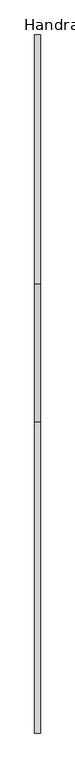
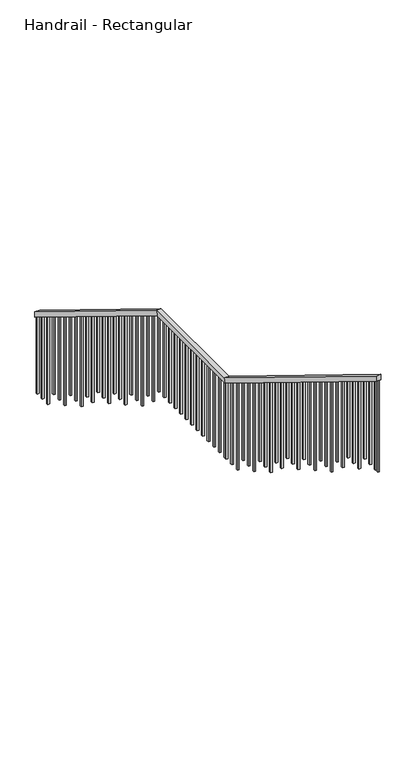
"""IFC4 building model written with IfcOpenShell, lengths in millimetres: railing geometry, Handrail - Rectangular."""

from ifc_helpers import new_model, si_unit, frame, origin, place, context, project, spatial, polyline, outline, extrude, faceted_brep, source, transform, mapped, element, save


def handrail_rectangular_7aeb163b(model_context):
    return source(origin(), model_context, "Body", "SolidModel", [
        faceted_brep([(2025.6499995, 20358.1, 10452.1), (2025.6499995, 20358.1, 10392.4981634), (1974.8499995, 20358.1, 10392.4981634), (1974.8499995, 20358.1, 10452.1), (2025.6499995, 18122.9, 11823.7), (2025.6499995, 18108.5562663, 11772.9), (1974.8499995, 18108.5562663, 11772.9), (1974.8499995, 18122.9, 11823.7), (2025.6499995, 16878.3, 11823.7), (2025.6499995, 16863.9562663, 11772.9), (1974.8499995, 16863.9562663, 11772.9), (1974.8499995, 16878.3, 11823.7), (2025.6499995, 14084.3, 13538.2), (1974.8499995, 14084.3, 13538.2), (1974.8499995, 14084.3, 13478.5981634), (2025.6499995, 14084.3, 13478.5981634)], [[[0, 1, 2, 3]], [[1, 0, 4, 5]], [[2, 1, 5, 6]], [[3, 2, 6, 7]], [[0, 3, 7, 4]], [[5, 4, 8, 9]], [[6, 5, 9, 10]], [[7, 6, 10, 11]], [[4, 7, 11, 8]], [[12, 13, 14, 15]], [[9, 8, 12, 15]], [[10, 9, 15, 14]], [[11, 10, 14, 13]], [[8, 11, 13, 12]]]),
        extrude(outline(polyline([(14144.625, 13441.5805498), (14144.625, 12452.35), (14125.575, 12452.35), (14125.575, 13453.2703225), (14144.625, 13441.5805498)])), frame((1990.7249995, 0.0, 0.0), z_axis=(1.0, 0.0, 0.0), x_axis=(0.0, 1.0, 0.0)), (0.0, 0.0, 1.0), 19.05),
        extrude(outline(polyline([(14246.225, 13379.2350952), (14246.225, 12452.35), (14227.175, 12452.35), (14227.175, 13390.9248679), (14246.225, 13379.2350952)])), frame((1990.7249995, 0.0, 0.0), z_axis=(1.0, 0.0, 0.0), x_axis=(0.0, 1.0, 0.0)), (0.0, 0.0, 1.0), 19.05),
        extrude(outline(polyline([(14347.825, 13316.8896407), (14347.825, 12452.35), (14328.775, 12452.35), (14328.775, 13328.5794134), (14347.825, 13316.8896407)])), frame((1990.7249995, 0.0, 0.0), z_axis=(1.0, 0.0, 0.0), x_axis=(0.0, 1.0, 0.0)), (0.0, 0.0, 1.0), 19.05),
        extrude(outline(polyline([(14449.425, 13254.5441861), (14449.425, 12280.9), (14430.375, 12280.9), (14430.375, 13266.2339589), (14449.425, 13254.5441861)])), frame((1990.7249995, 0.0, 0.0), z_axis=(1.0, 0.0, 0.0), x_axis=(0.0, 1.0, 0.0)), (0.0, 0.0, 1.0), 19.05),
        extrude(outline(polyline([(14551.025, 13192.1987316), (14551.025, 12280.9), (14531.975, 12280.9), (14531.975, 13203.8885043), (14551.025, 13192.1987316)])), frame((1990.7249995, 0.0, 0.0), z_axis=(1.0, 0.0, 0.0), x_axis=(0.0, 1.0, 0.0)), (0.0, 0.0, 1.0), 19.05),
        extrude(outline(polyline([(14652.625, 13129.853277), (14652.625, 12280.9), (14633.575, 12280.9), (14633.575, 13141.5430498), (14652.625, 13129.853277)])), frame((1990.7249995, 0.0, 0.0), z_axis=(1.0, 0.0, 0.0), x_axis=(0.0, 1.0, 0.0)), (0.0, 0.0, 1.0), 19.05),
        extrude(outline(polyline([(14754.225, 13067.5078225), (14754.225, 12109.45), (14735.175, 12109.45), (14735.175, 13079.1975952), (14754.225, 13067.5078225)])), frame((1990.7249995, 0.0, 0.0), z_axis=(1.0, 0.0, 0.0), x_axis=(0.0, 1.0, 0.0)), (0.0, 0.0, 1.0), 19.05),
        extrude(outline(polyline([(14855.825, 13005.1623679), (14855.825, 12109.45), (14836.775, 12109.45), (14836.775, 13016.8521407), (14855.825, 13005.1623679)])), frame((1990.7249995, 0.0, 0.0), z_axis=(1.0, 0.0, 0.0), x_axis=(0.0, 1.0, 0.0)), (0.0, 0.0, 1.0), 19.05),
        extrude(outline(polyline([(14957.425, 12942.8169134), (14957.425, 11938.0), (14938.375, 11938.0), (14938.375, 12954.5066861), (14957.425, 12942.8169134)])), frame((1990.7249995, 0.0, 0.0), z_axis=(1.0, 0.0, 0.0), x_axis=(0.0, 1.0, 0.0)), (0.0, 0.0, 1.0), 19.05),
        extrude(outline(polyline([(15059.025, 12880.4714589), (15059.025, 11938.0), (15039.975, 11938.0), (15039.975, 12892.1612316), (15059.025, 12880.4714589)])), frame((1990.7249995, 0.0, 0.0), z_axis=(1.0, 0.0, 0.0), x_axis=(0.0, 1.0, 0.0)), (0.0, 0.0, 1.0), 19.05),
        extrude(outline(polyline([(15160.625, 12818.1260043), (15160.625, 11938.0), (15141.575, 11938.0), (15141.575, 12829.815777), (15160.625, 12818.1260043)])), frame((1990.7249995, 0.0, 0.0), z_axis=(1.0, 0.0, 0.0), x_axis=(0.0, 1.0, 0.0)), (0.0, 0.0, 1.0), 19.05),
        extrude(outline(polyline([(15262.225, 12755.7805498), (15262.225, 11766.55), (15243.175, 11766.55), (15243.175, 12767.4703225), (15262.225, 12755.7805498)])), frame((1990.7249995, 0.0, 0.0), z_axis=(1.0, 0.0, 0.0), x_axis=(0.0, 1.0, 0.0)), (0.0, 0.0, 1.0), 19.05),
        extrude(outline(polyline([(15363.825, 12693.4350952), (15363.825, 11766.55), (15344.775, 11766.55), (15344.775, 12705.1248679), (15363.825, 12693.4350952)])), frame((1990.7249995, 0.0, 0.0), z_axis=(1.0, 0.0, 0.0), x_axis=(0.0, 1.0, 0.0)), (0.0, 0.0, 1.0), 19.05),
        extrude(outline(polyline([(15465.425, 12631.0896407), (15465.425, 11766.55), (15446.375, 11766.55), (15446.375, 12642.7794134), (15465.425, 12631.0896407)])), frame((1990.7249995, 0.0, 0.0), z_axis=(1.0, 0.0, 0.0), x_axis=(0.0, 1.0, 0.0)), (0.0, 0.0, 1.0), 19.05),
        extrude(outline(polyline([(15567.025, 12568.7441861), (15567.025, 11595.1), (15547.975, 11595.1), (15547.975, 12580.4339589), (15567.025, 12568.7441861)])), frame((1990.7249995, 0.0, 0.0), z_axis=(1.0, 0.0, 0.0), x_axis=(0.0, 1.0, 0.0)), (0.0, 0.0, 1.0), 19.05),
        extrude(outline(polyline([(15668.625, 12506.3987316), (15668.625, 11595.1), (15649.575, 11595.1), (15649.575, 12518.0885043), (15668.625, 12506.3987316)])), frame((1990.7249995, 0.0, 0.0), z_axis=(1.0, 0.0, 0.0), x_axis=(0.0, 1.0, 0.0)), (0.0, 0.0, 1.0), 19.05),
        extrude(outline(polyline([(15770.225, 12444.053277), (15770.225, 11595.1), (15751.175, 11595.1), (15751.175, 12455.7430498), (15770.225, 12444.053277)])), frame((1990.7249995, 0.0, 0.0), z_axis=(1.0, 0.0, 0.0), x_axis=(0.0, 1.0, 0.0)), (0.0, 0.0, 1.0), 19.05),
        extrude(outline(polyline([(15871.825, 12381.7078225), (15871.825, 11423.65), (15852.775, 11423.65), (15852.775, 12393.3975952), (15871.825, 12381.7078225)])), frame((1990.7249995, 0.0, 0.0), z_axis=(1.0, 0.0, 0.0), x_axis=(0.0, 1.0, 0.0)), (0.0, 0.0, 1.0), 19.05),
        extrude(outline(polyline([(15973.425, 12319.3623679), (15973.425, 11423.65), (15954.375, 11423.65), (15954.375, 12331.0521407), (15973.425, 12319.3623679)])), frame((1990.7249995, 0.0, 0.0), z_axis=(1.0, 0.0, 0.0), x_axis=(0.0, 1.0, 0.0)), (0.0, 0.0, 1.0), 19.05),
        extrude(outline(polyline([(16075.025, 12257.0169134), (16075.025, 11252.2), (16055.975, 11252.2), (16055.975, 12268.7066861), (16075.025, 12257.0169134)])), frame((1990.7249995, 0.0, 0.0), z_axis=(1.0, 0.0, 0.0), x_axis=(0.0, 1.0, 0.0)), (0.0, 0.0, 1.0), 19.05),
        extrude(outline(polyline([(16176.625, 12194.6714589), (16176.625, 11252.2), (16157.575, 11252.2), (16157.575, 12206.3612316), (16176.625, 12194.6714589)])), frame((1990.7249995, 0.0, 0.0), z_axis=(1.0, 0.0, 0.0), x_axis=(0.0, 1.0, 0.0)), (0.0, 0.0, 1.0), 19.05),
        extrude(outline(polyline([(16278.225, 12132.3260043), (16278.225, 11252.2), (16259.175, 11252.2), (16259.175, 12144.015777), (16278.225, 12132.3260043)])), frame((1990.7249995, 0.0, 0.0), z_axis=(1.0, 0.0, 0.0), x_axis=(0.0, 1.0, 0.0)), (0.0, 0.0, 1.0), 19.05),
        extrude(outline(polyline([(16379.825, 12069.9805498), (16379.825, 11080.75), (16360.775, 11080.75), (16360.775, 12081.6703225), (16379.825, 12069.9805498)])), frame((1990.7249995, 0.0, 0.0), z_axis=(1.0, 0.0, 0.0), x_axis=(0.0, 1.0, 0.0)), (0.0, 0.0, 1.0), 19.05),
        extrude(outline(polyline([(16481.425, 12007.6350952), (16481.425, 11080.75), (16462.375, 11080.75), (16462.375, 12019.3248679), (16481.425, 12007.6350952)])), frame((1990.7249995, 0.0, 0.0), z_axis=(1.0, 0.0, 0.0), x_axis=(0.0, 1.0, 0.0)), (0.0, 0.0, 1.0), 19.05),
        extrude(outline(polyline([(16583.025, 11945.2896407), (16583.025, 11080.75), (16563.975, 11080.75), (16563.975, 11956.9794134), (16583.025, 11945.2896407)])), frame((1990.7249995, 0.0, 0.0), z_axis=(1.0, 0.0, 0.0), x_axis=(0.0, 1.0, 0.0)), (0.0, 0.0, 1.0), 19.05),
        extrude(outline(polyline([(16684.625, 11882.9441861), (16684.625, 10909.3), (16665.575, 10909.3), (16665.575, 11894.6339589), (16684.625, 11882.9441861)])), frame((1990.7249995, 0.0, 0.0), z_axis=(1.0, 0.0, 0.0), x_axis=(0.0, 1.0, 0.0)), (0.0, 0.0, 1.0), 19.05),
        extrude(outline(polyline([(16786.225, 11820.5987316), (16786.225, 10909.3), (16767.175, 10909.3), (16767.175, 11832.2885043), (16786.225, 11820.5987316)])), frame((1990.7249995, 0.0, 0.0), z_axis=(1.0, 0.0, 0.0), x_axis=(0.0, 1.0, 0.0)), (0.0, 0.0, 1.0), 19.05),
        extrude(outline(polyline([(2009.7749995, 16913.225), (2009.7749995, 16894.175), (1990.7249995, 16894.175), (1990.7249995, 16913.225), (2009.7749995, 16913.225)])), frame((0.0, 0.0, 10909.3), z_axis=(0.0, 0.0, 1.0), x_axis=(1.0, 0.0, 0.0)), (0.0, 0.0, 1.0), 863.6),
        extrude(outline(polyline([(2009.7749995, 17014.825), (2009.7749995, 16995.775), (1990.7249995, 16995.775), (1990.7249995, 17014.825), (2009.7749995, 17014.825)])), frame((0.0, 0.0, 10909.3), z_axis=(0.0, 0.0, 1.0), x_axis=(1.0, 0.0, 0.0)), (0.0, 0.0, 1.0), 863.6),
        extrude(outline(polyline([(2009.7749995, 17116.425), (2009.7749995, 17097.375), (1990.7249995, 17097.375), (1990.7249995, 17116.425), (2009.7749995, 17116.425)])), frame((0.0, 0.0, 10909.3), z_axis=(0.0, 0.0, 1.0), x_axis=(1.0, 0.0, 0.0)), (0.0, 0.0, 1.0), 863.6),
        extrude(outline(polyline([(2009.7749995, 17218.025), (2009.7749995, 17198.975), (1990.7249995, 17198.975), (1990.7249995, 17218.025), (2009.7749995, 17218.025)])), frame((0.0, 0.0, 10909.3), z_axis=(0.0, 0.0, 1.0), x_axis=(1.0, 0.0, 0.0)), (0.0, 0.0, 1.0), 863.6),
        extrude(outline(polyline([(2009.7749995, 17319.625), (2009.7749995, 17300.575), (1990.7249995, 17300.575), (1990.7249995, 17319.625), (2009.7749995, 17319.625)])), frame((0.0, 0.0, 10909.3), z_axis=(0.0, 0.0, 1.0), x_axis=(1.0, 0.0, 0.0)), (0.0, 0.0, 1.0), 863.6),
        extrude(outline(polyline([(2009.7749995, 17421.225), (2009.7749995, 17402.175), (1990.7249995, 17402.175), (1990.7249995, 17421.225), (2009.7749995, 17421.225)])), frame((0.0, 0.0, 10909.3), z_axis=(0.0, 0.0, 1.0), x_axis=(1.0, 0.0, 0.0)), (0.0, 0.0, 1.0), 863.6),
        extrude(outline(polyline([(2009.7749995, 17522.825), (2009.7749995, 17503.775), (1990.7249995, 17503.775), (1990.7249995, 17522.825), (2009.7749995, 17522.825)])), frame((0.0, 0.0, 10909.3), z_axis=(0.0, 0.0, 1.0), x_axis=(1.0, 0.0, 0.0)), (0.0, 0.0, 1.0), 863.6),
        extrude(outline(polyline([(2009.7749995, 17624.425), (2009.7749995, 17605.375), (1990.7249995, 17605.375), (1990.7249995, 17624.425), (2009.7749995, 17624.425)])), frame((0.0, 0.0, 10909.3), z_axis=(0.0, 0.0, 1.0), x_axis=(1.0, 0.0, 0.0)), (0.0, 0.0, 1.0), 863.6),
        extrude(outline(polyline([(2009.7749995, 17726.025), (2009.7749995, 17706.975), (1990.7249995, 17706.975), (1990.7249995, 17726.025), (2009.7749995, 17726.025)])), frame((0.0, 0.0, 10909.3), z_axis=(0.0, 0.0, 1.0), x_axis=(1.0, 0.0, 0.0)), (0.0, 0.0, 1.0), 863.6),
        extrude(outline(polyline([(2009.7749995, 17827.625), (2009.7749995, 17808.575), (1990.7249995, 17808.575), (1990.7249995, 17827.625), (2009.7749995, 17827.625)])), frame((0.0, 0.0, 10909.3), z_axis=(0.0, 0.0, 1.0), x_axis=(1.0, 0.0, 0.0)), (0.0, 0.0, 1.0), 863.6),
        extrude(outline(polyline([(2009.7749995, 17929.225), (2009.7749995, 17910.175), (1990.7249995, 17910.175), (1990.7249995, 17929.225), (2009.7749995, 17929.225)])), frame((0.0, 0.0, 10909.3), z_axis=(0.0, 0.0, 1.0), x_axis=(1.0, 0.0, 0.0)), (0.0, 0.0, 1.0), 863.6),
        extrude(outline(polyline([(2009.7749995, 18030.825), (2009.7749995, 18011.775), (1990.7249995, 18011.775), (1990.7249995, 18030.825), (2009.7749995, 18030.825)])), frame((0.0, 0.0, 10909.3), z_axis=(0.0, 0.0, 1.0), x_axis=(1.0, 0.0, 0.0)), (0.0, 0.0, 1.0), 863.6),
        extrude(outline(polyline([(18234.025, 11695.9078225), (18234.025, 10737.85), (18214.975, 10737.85), (18214.975, 11707.5975952), (18234.025, 11695.9078225)])), frame((1990.7249995, 0.0, 0.0), z_axis=(1.0, 0.0, 0.0), x_axis=(0.0, 1.0, 0.0)), (0.0, 0.0, 1.0), 19.05),
        extrude(outline(polyline([(18335.625, 11633.5623679), (18335.625, 10737.85), (18316.575, 10737.85), (18316.575, 11645.2521407), (18335.625, 11633.5623679)])), frame((1990.7249995, 0.0, 0.0), z_axis=(1.0, 0.0, 0.0), x_axis=(0.0, 1.0, 0.0)), (0.0, 0.0, 1.0), 19.05),
        extrude(outline(polyline([(18437.225, 11571.2169134), (18437.225, 10566.4), (18418.175, 10566.4), (18418.175, 11582.9066861), (18437.225, 11571.2169134)])), frame((1990.7249995, 0.0, 0.0), z_axis=(1.0, 0.0, 0.0), x_axis=(0.0, 1.0, 0.0)), (0.0, 0.0, 1.0), 19.05),
        extrude(outline(polyline([(18538.825, 11508.8714589), (18538.825, 10566.4), (18519.775, 10566.4), (18519.775, 11520.5612316), (18538.825, 11508.8714589)])), frame((1990.7249995, 0.0, 0.0), z_axis=(1.0, 0.0, 0.0), x_axis=(0.0, 1.0, 0.0)), (0.0, 0.0, 1.0), 19.05),
        extrude(outline(polyline([(18640.425, 11446.5260043), (18640.425, 10566.4), (18621.375, 10566.4), (18621.375, 11458.215777), (18640.425, 11446.5260043)])), frame((1990.7249995, 0.0, 0.0), z_axis=(1.0, 0.0, 0.0), x_axis=(0.0, 1.0, 0.0)), (0.0, 0.0, 1.0), 19.05),
        extrude(outline(polyline([(18742.025, 11384.1805498), (18742.025, 10394.95), (18722.975, 10394.95), (18722.975, 11395.8703225), (18742.025, 11384.1805498)])), frame((1990.7249995, 0.0, 0.0), z_axis=(1.0, 0.0, 0.0), x_axis=(0.0, 1.0, 0.0)), (0.0, 0.0, 1.0), 19.05),
        extrude(outline(polyline([(18843.625, 11321.8350952), (18843.625, 10394.95), (18824.575, 10394.95), (18824.575, 11333.5248679), (18843.625, 11321.8350952)])), frame((1990.7249995, 0.0, 0.0), z_axis=(1.0, 0.0, 0.0), x_axis=(0.0, 1.0, 0.0)), (0.0, 0.0, 1.0), 19.05),
        extrude(outline(polyline([(18945.225, 11259.4896407), (18945.225, 10394.95), (18926.175, 10394.95), (18926.175, 11271.1794134), (18945.225, 11259.4896407)])), frame((1990.7249995, 0.0, 0.0), z_axis=(1.0, 0.0, 0.0), x_axis=(0.0, 1.0, 0.0)), (0.0, 0.0, 1.0), 19.05),
        extrude(outline(polyline([(19046.825, 11197.1441861), (19046.825, 10223.5), (19027.775, 10223.5), (19027.775, 11208.8339589), (19046.825, 11197.1441861)])), frame((1990.7249995, 0.0, 0.0), z_axis=(1.0, 0.0, 0.0), x_axis=(0.0, 1.0, 0.0)), (0.0, 0.0, 1.0), 19.05),
        extrude(outline(polyline([(19148.425, 11134.7987316), (19148.425, 10223.5), (19129.375, 10223.5), (19129.375, 11146.4885043), (19148.425, 11134.7987316)])), frame((1990.7249995, 0.0, 0.0), z_axis=(1.0, 0.0, 0.0), x_axis=(0.0, 1.0, 0.0)), (0.0, 0.0, 1.0), 19.05),
        extrude(outline(polyline([(19250.025, 11072.453277), (19250.025, 10223.5), (19230.975, 10223.5), (19230.975, 11084.1430498), (19250.025, 11072.453277)])), frame((1990.7249995, 0.0, 0.0), z_axis=(1.0, 0.0, 0.0), x_axis=(0.0, 1.0, 0.0)), (0.0, 0.0, 1.0), 19.05),
        extrude(outline(polyline([(19351.625, 11010.1078225), (19351.625, 10052.05), (19332.575, 10052.05), (19332.575, 11021.7975952), (19351.625, 11010.1078225)])), frame((1990.7249995, 0.0, 0.0), z_axis=(1.0, 0.0, 0.0), x_axis=(0.0, 1.0, 0.0)), (0.0, 0.0, 1.0), 19.05),
        extrude(outline(polyline([(19453.225, 10947.7623679), (19453.225, 10052.05), (19434.175, 10052.05), (19434.175, 10959.4521407), (19453.225, 10947.7623679)])), frame((1990.7249995, 0.0, 0.0), z_axis=(1.0, 0.0, 0.0), x_axis=(0.0, 1.0, 0.0)), (0.0, 0.0, 1.0), 19.05),
        extrude(outline(polyline([(19554.825, 10885.4169134), (19554.825, 9880.6), (19535.775, 9880.6), (19535.775, 10897.1066861), (19554.825, 10885.4169134)])), frame((1990.7249995, 0.0, 0.0), z_axis=(1.0, 0.0, 0.0), x_axis=(0.0, 1.0, 0.0)), (0.0, 0.0, 1.0), 19.05),
        extrude(outline(polyline([(19656.425, 10823.0714589), (19656.425, 9880.6), (19637.375, 9880.6), (19637.375, 10834.7612316), (19656.425, 10823.0714589)])), frame((1990.7249995, 0.0, 0.0), z_axis=(1.0, 0.0, 0.0), x_axis=(0.0, 1.0, 0.0)), (0.0, 0.0, 1.0), 19.05),
        extrude(outline(polyline([(19758.025, 10760.7260043), (19758.025, 9880.6), (19738.975, 9880.6), (19738.975, 10772.415777), (19758.025, 10760.7260043)])), frame((1990.7249995, 0.0, 0.0), z_axis=(1.0, 0.0, 0.0), x_axis=(0.0, 1.0, 0.0)), (0.0, 0.0, 1.0), 19.05),
        extrude(outline(polyline([(19859.625, 10698.3805498), (19859.625, 9709.15), (19840.575, 9709.15), (19840.575, 10710.0703225), (19859.625, 10698.3805498)])), frame((1990.7249995, 0.0, 0.0), z_axis=(1.0, 0.0, 0.0), x_axis=(0.0, 1.0, 0.0)), (0.0, 0.0, 1.0), 19.05),
        extrude(outline(polyline([(19961.225, 10636.0350952), (19961.225, 9709.15), (19942.175, 9709.15), (19942.175, 10647.7248679), (19961.225, 10636.0350952)])), frame((1990.7249995, 0.0, 0.0), z_axis=(1.0, 0.0, 0.0), x_axis=(0.0, 1.0, 0.0)), (0.0, 0.0, 1.0), 19.05),
        extrude(outline(polyline([(20062.825, 10573.6896407), (20062.825, 9709.15), (20043.775, 9709.15), (20043.775, 10585.3794134), (20062.825, 10573.6896407)])), frame((1990.7249995, 0.0, 0.0), z_axis=(1.0, 0.0, 0.0), x_axis=(0.0, 1.0, 0.0)), (0.0, 0.0, 1.0), 19.05),
        extrude(outline(polyline([(20164.425, 10511.3441861), (20164.425, 9537.7), (20145.375, 9537.7), (20145.375, 10523.0339589), (20164.425, 10511.3441861)])), frame((1990.7249995, 0.0, 0.0), z_axis=(1.0, 0.0, 0.0), x_axis=(0.0, 1.0, 0.0)), (0.0, 0.0, 1.0), 19.05),
        extrude(outline(polyline([(20266.025, 10448.9987316), (20266.025, 9537.7), (20246.975, 9537.7), (20246.975, 10460.6885043), (20266.025, 10448.9987316)])), frame((1990.7249995, 0.0, 0.0), z_axis=(1.0, 0.0, 0.0), x_axis=(0.0, 1.0, 0.0)), (0.0, 0.0, 1.0), 19.05),
        extrude(outline(polyline([(2009.7749995, 16887.825), (2009.7749995, 16868.775), (1990.7249995, 16868.775), (1990.7249995, 16887.825), (2009.7749995, 16887.825)])), frame((0.0, 0.0, 10909.3), z_axis=(0.0, 0.0, 1.0), x_axis=(1.0, 0.0, 0.0)), (0.0, 0.0, 1.0), 863.6),
        extrude(outline(polyline([(18132.425, 11758.253277), (18132.425, 10909.3), (18113.375, 10909.3), (18113.375, 11769.9430498), (18132.425, 11758.253277)])), frame((1990.7249995, 0.0, 0.0), z_axis=(1.0, 0.0, 0.0), x_axis=(0.0, 1.0, 0.0)), (0.0, 0.0, 1.0), 19.05),
        extrude(outline(polyline([(14103.35, 13466.9083907), (14103.35, 12452.35), (14084.3, 12452.35), (14084.3, 13478.5981634), (14103.35, 13466.9083907)])), frame((1990.7249995, 0.0, 0.0), z_axis=(1.0, 0.0, 0.0), x_axis=(0.0, 1.0, 0.0)), (0.0, 0.0, 1.0), 19.05),
        extrude(outline(polyline([(20358.1, 10392.4981634), (20358.1, 9537.7), (20339.05, 9537.7), (20339.05, 10404.1879361), (20358.1, 10392.4981634)])), frame((1990.7249995, 0.0, 0.0), z_axis=(1.0, 0.0, 0.0), x_axis=(0.0, 1.0, 0.0)), (0.0, 0.0, 1.0), 19.05),
    ])


if __name__ == "__main__":
    model = new_model("IFC4")
    model_context = context("Model", 3, world=origin())
    ifc_project = project(units=[si_unit("LENGTHUNIT", "METRE", prefix="MILLI")], contexts=[model_context])
    site = spatial("IfcSite", under=ifc_project)
    building = spatial("IfcBuilding", under=site)
    placement = place(None, origin())
    handrail_rectangular_shape = handrail_rectangular_7aeb163b(model_context)
    element("IfcRailing", 1, ObjectType="Handrail - Rectangular", at=placement, inside=building, context=model_context, shape_type="MappedRepresentation", body=[
        mapped(handrail_rectangular_shape, transform((0.0, 0.0, 0.0), x_axis=(1.0, 0.0, 0.0), y_axis=(0.0, 1.0, 0.0), z_axis=(0.0, 0.0, 1.0))),
    ])
    save(model, "model.ifc")
